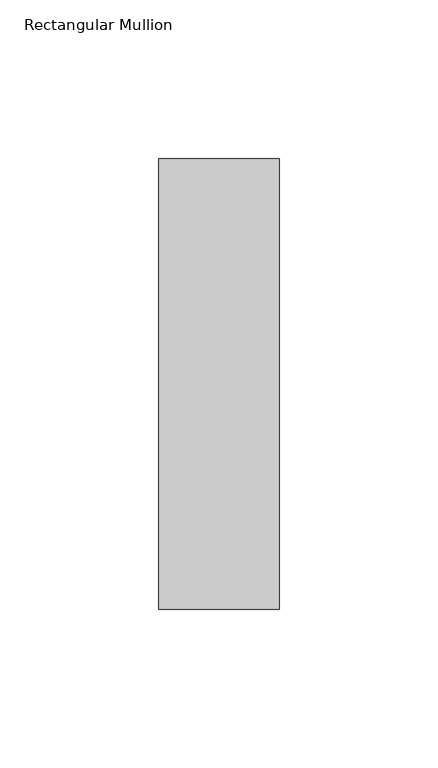
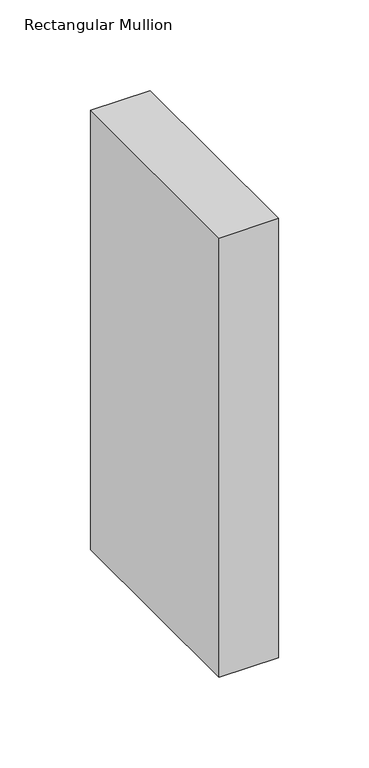
"""IFC4 building model written with IfcOpenShell, lengths in millimetres: member geometry, Rectangular Mullion : NLRS_21_CWM_hsb-regel 38x142_gen_rsf."""

from ifc_helpers import new_model, si_unit, frame, origin, place, context, project, spatial, polyline, outline, extrude, source, transform, mapped, element, save


def rectangular_mullion_90e0555f(model_context):
    return source(origin(), model_context, "Body", "SweptSolid", [
        extrude(outline(polyline([(-38.0, -71.0), (-38.0, 71.0), (0.0, 71.0), (0.0, -71.0), (-38.0, -71.0)])), frame((0.0, 0.0, -296.0), z_axis=(0.0, 0.0, 1.0), x_axis=(1.0, 0.0, 0.0)), (0.0, 0.0, 1.0), 296.0),
    ])


if __name__ == "__main__":
    model = new_model("IFC4")
    model_context = context("Model", 3, world=origin())
    ifc_project = project(units=[si_unit("LENGTHUNIT", "METRE", prefix="MILLI")], contexts=[model_context])
    site = spatial("IfcSite", under=ifc_project)
    building = spatial("IfcBuilding", under=site)
    placement = place(None, origin())
    rectangular_mullion_shape = rectangular_mullion_90e0555f(model_context)
    element("IfcMember", 1, ObjectType="Rectangular Mullion : NLRS_21_CWM_hsb-regel 38x142_gen_rsf", at=placement, inside=building, context=model_context, shape_type="MappedRepresentation", body=[
        mapped(rectangular_mullion_shape, transform((0.0, 0.0, 0.0), x_axis=(1.0, 0.0, 0.0), y_axis=(0.0, 1.0, 0.0), z_axis=(0.0, 0.0, 1.0))),
    ])
    save(model, "model.ifc")

# Revit data of these elements
# Type "Rectangular Mullion : NLRS_21_CWM_hsb-regel 38x142_gen_rsf"
#   Export Type to IFC As = "IfcWall"
#   Type IfcGUID = "07M7mRoiH1CR8m_RSKIwpF"
#   Assembly Code = "21.10"
#   built-in parameter 1007322 = 0.465879 (stored number, unit not read)
#   built-in parameter 1007321 = 0.062336 (stored number, unit not read)
#   built-in parameter 1007320 = 0.062336 (stored number, unit not read)
# Element 1 (IfcMember, "Rectangular Mullion : NLRS_21_CWM_hsb-regel 38x142_gen_rsf")
#   Materials on its faces: "NLRS_i2_hout naaldhout vuren_gen_rsf"
# Materials
#   "NLRS_i2_hout naaldhout vuren_gen_rsf": class "I - Hout", colour RGB 234 199 147, transparency 0, Keynote = "i2", Manufacturer = "Revit Standards Foundation", URL = "www.revitstandards.org", Description = "hout vuren", Cost = 0
